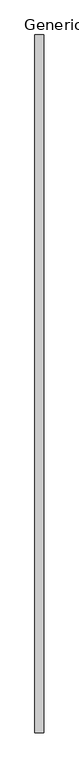
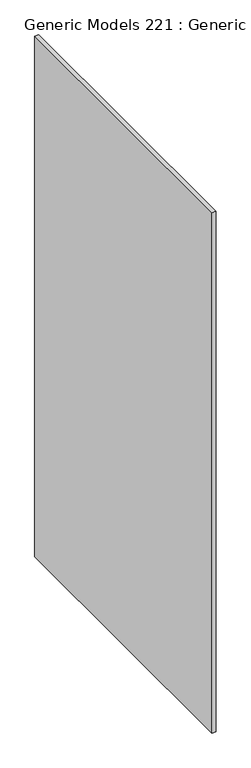
"""IFC4 building model written with IfcOpenShell, lengths in millimetres: proxy geometry, Generic Models 221 : Generic Models 1."""

from ifc_helpers import new_model, si_unit, frame, origin, place, context, project, spatial, polyline, outline, extrude, source, transform, mapped, element, save


def generic_models_221_generic_models_1_b97a9e7e(model_context):
    return source(origin(), model_context, "Body", "SweptSolid", [
        extrude(outline(polyline([(46142.275, 1219.2), (46142.275, 0.0), (46126.4, 0.0), (46126.4, 1219.2), (46142.275, 1219.2)])), frame((0.0, 0.0, 6.35), z_axis=(0.0, 0.0, 1.0), x_axis=(1.0, 0.0, 0.0)), (0.0, 0.0, 1.0), 2181.8704978),
    ])


if __name__ == "__main__":
    model = new_model("IFC4")
    model_context = context("Model", 3, world=origin())
    ifc_project = project(units=[si_unit("LENGTHUNIT", "METRE", prefix="MILLI")], contexts=[model_context])
    site = spatial("IfcSite", under=ifc_project)
    building = spatial("IfcBuilding", under=site)
    placement = place(None, origin())
    generic_models_221_generic_models_1_shape = generic_models_221_generic_models_1_b97a9e7e(model_context)
    element("IfcBuildingElementProxy", 1, Name="Generic Models 221 : Generic Models 1", ObjectType="Generic Models 221 : Generic Models 1", at=placement, inside=building, context=model_context, shape_type="MappedRepresentation", body=[
        mapped(generic_models_221_generic_models_1_shape, transform((0.0, 0.0, 0.0), x_axis=(1.0, 0.0, 0.0), y_axis=(0.0, 1.0, 0.0), z_axis=(0.0, 0.0, 1.0))),
    ])
    save(model, "model.ifc")

# Revit data of these elements
# Element 1 (IfcBuildingElementProxy, "Generic Models 221 : Generic Models 1")
#   Materials on its faces: "GYP. BD (SEE 'WALL TAG' & 'LAYER MATERIAL SCHEDULE' FOR DETAILS)"
# Materials
#   "GYP. BD (SEE 'WALL TAG' & 'LAYER MATERIAL SCHEDULE' FOR DETAILS)": class "Generic", colour RGB 237 236 233, transparency 0, Description = "Gypsum Wall Board", Cost = 0
